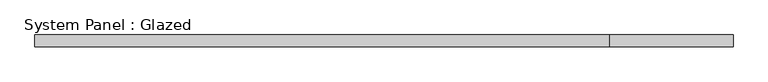
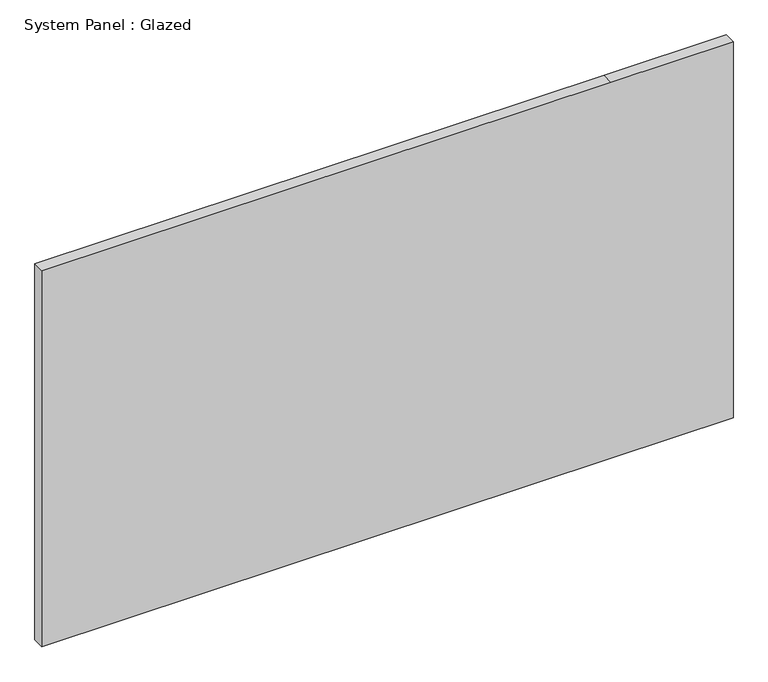
"""IFC4 building model written with IfcOpenShell, lengths in millimetres: plate geometry, System Panel : Glazed."""

from ifc_helpers import new_model, si_unit, frame, origin, place, context, project, spatial, polyline, outline, extrude, source, transform, mapped, element, save


def system_panel_glazed_f4fcbcda(model_context):
    return source(origin(), model_context, "Body", "SweptSolid", [
        extrude(outline(polyline([(0.0, -756.44375), (0.0, 488.95), (0.0, 756.44375), (869.95, 756.44375), (869.95, 488.95), (869.95, -756.44375), (0.0, -756.44375)])), frame((0.0, -44.45, 0.0), z_axis=(0.0, 1.0, 0.0), x_axis=(0.0, 0.0, 1.0)), (0.0, 0.0, 1.0), 25.4),
    ])


if __name__ == "__main__":
    model = new_model("IFC4")
    model_context = context("Model", 3, world=origin())
    ifc_project = project(units=[si_unit("LENGTHUNIT", "METRE", prefix="MILLI")], contexts=[model_context])
    site = spatial("IfcSite", under=ifc_project)
    building = spatial("IfcBuilding", under=site)
    placement = place(None, origin())
    system_panel_glazed_shape = system_panel_glazed_f4fcbcda(model_context)
    element("IfcPlate", 1, ObjectType="System Panel : Glazed", at=placement, inside=building, context=model_context, shape_type="MappedRepresentation", body=[
        mapped(system_panel_glazed_shape, transform((0.0, 0.0, 0.0), x_axis=(1.0, 0.0, 0.0), y_axis=(0.0, 1.0, 0.0), z_axis=(0.0, 0.0, 1.0))),
    ])
    save(model, "model.ifc")

# Revit data of these elements
# Element 1 (IfcPlate, "System Panel : Glazed")
#   Materials on its faces: "Glass"
# Materials
#   "Glass": class "Glass", colour RGB 0 128 192, transparency 0.75
